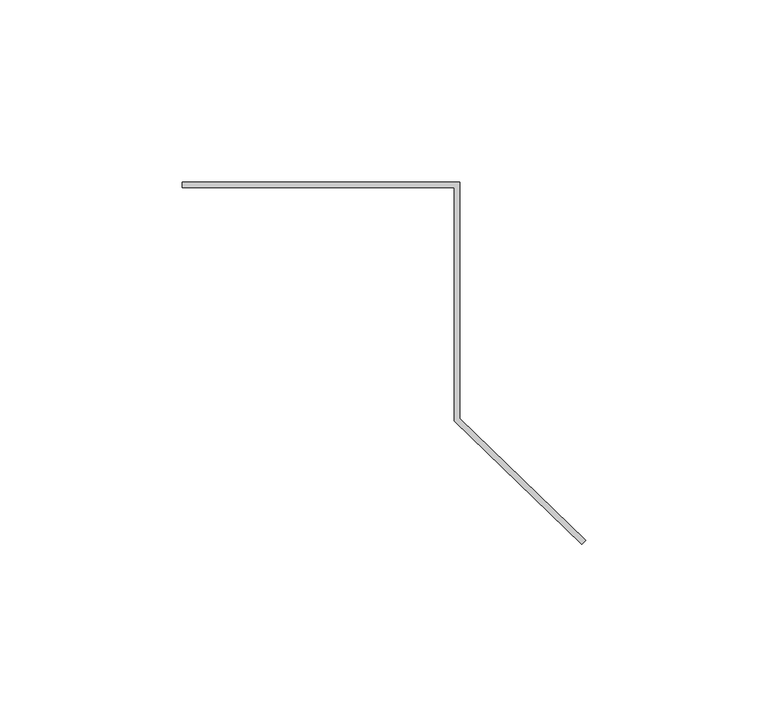
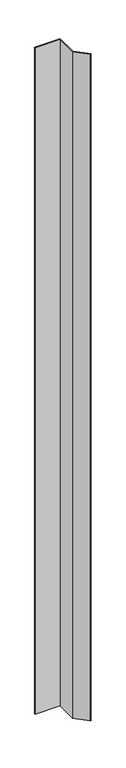
"""IFC4 building model written with IfcOpenShell, lengths in millimetres: proxy geometry, Generic Models 2:Generic Models 2:310765:Generic Models 2:310765 : Generic Models 2:Generic Models 2:310765:61 : Generic Models 2:Generic Models 2:310765:Generic Models 2:310765 : Generic Models 2:Generic Models 2:310765:300385."""

from ifc_helpers import new_model, si_unit, frame, origin, place, context, project, spatial, polyline, outline, extrude, source, transform, mapped, element, save


def generic_models_f5275963(model_context):
    return source(origin(), model_context, "Body", "SweptSolid", [
        extrude(outline(polyline([(667210.7617239, -568274.0939933), (667286.9617239, -568274.0939933), (667286.9617239, -568339.0177162), (667321.5133229, -568372.5097328), (667320.3906548, -568373.6324009), (667285.3742239, -568339.6898072), (667285.3742239, -568275.6814933), (667210.7617239, -568275.6814933), (667210.7617239, -568274.0939933)])), frame((0.0, 0.0, 4033.8810286), z_axis=(0.0, 0.0, 1.0), x_axis=(1.0, 0.0, 0.0)), (0.0, 0.0, 1.0), 2100.2189714),
    ])


if __name__ == "__main__":
    model = new_model("IFC4")
    model_context = context("Model", 3, world=origin())
    ifc_project = project(units=[si_unit("LENGTHUNIT", "METRE", prefix="MILLI")], contexts=[model_context])
    site = spatial("IfcSite", under=ifc_project)
    building = spatial("IfcBuilding", under=site)
    placement = place(None, origin())
    generic_models_shape = generic_models_f5275963(model_context)
    element("IfcBuildingElementProxy", 1, Name="Generic Models 2:Generic Models 2:310765:Generic Models 2:310765 : Generic Models 2:Generic Models 2:310765:61 : Generic Models 2:Generic Models 2:310765:Generic Models 2:310765 : Generic Models 2:Generic Models 2:310765:300385", ObjectType="Generic Models 2:Generic Models 2:310765:Generic Models 2:310765 : Generic Models 2:Generic Models 2:310765:61 : Generic Models 2:Generic Models 2:310765:Generic Models 2:310765 : Generic Models 2:Generic Models 2:310765:300385", at=placement, inside=building, context=model_context, shape_type="MappedRepresentation", body=[
        mapped(generic_models_shape, transform((0.0, 0.0, 0.0), x_axis=(1.0, 0.0, 0.0), y_axis=(0.0, 1.0, 0.0), z_axis=(0.0, 0.0, 1.0))),
    ])
    save(model, "model.ifc")

# Revit data of these elements
# Type "Generic Models 2:Generic Models 2:310765:Generic Models 2:310765 : Generic Models 2:Generic Models 2:310765:61 : Generic Models 2:Generic Models 2:310765:Generic Models 2:310765 : Generic Models 2:Generic Models 2:310765:300385"
#   NameOverride = "Generic Models 2:Generic Models 2:310765:Generic Models 2:310765 : Generic Models 2:Generic Models 2:310765:300385"
#   ObjectTypeOverride = "Generic Models 2:310765 : Generic Models 2:Generic Models 2:310765"
#   Reference = "Generic Models 2"
#   Tag = "300385"
# Element 1 (IfcBuildingElementProxy, "Generic Models 2:Generic Models 2:310765:Generic Models 2:310765 : Generic Models 2:Generic Models 2:310765:61 : Generic Models 2:Generic Models 2:310765:Generic Models 2:310765 : Generic Models 2:Generic Models 2:310765:300385")
#   Materials on its faces: "BRAKE METAL CLOSURE TRIM"
# Materials
#   "BRAKE METAL CLOSURE TRIM": class "Unassigned", colour RGB 210 209 208, transparency 0, Cost = 0
